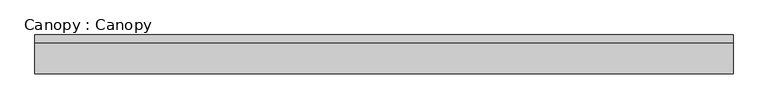
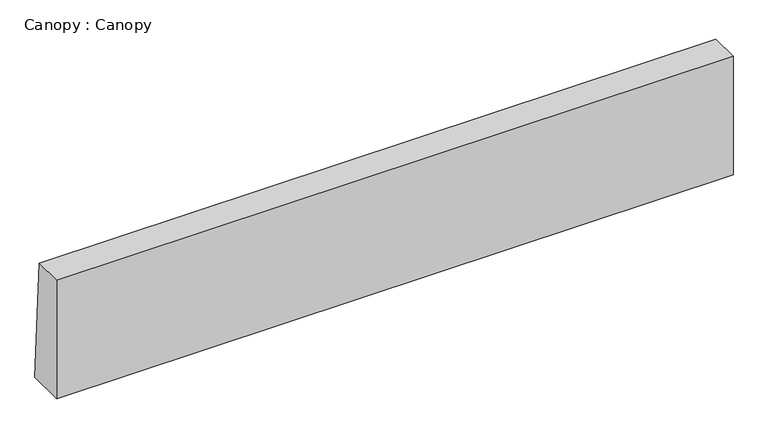
"""IFC4 building model written with IfcOpenShell, lengths in millimetres: proxy geometry, Canopy : Canopy."""

from ifc_helpers import new_model, si_unit, frame, origin, place, context, project, spatial, polyline, outline, extrude, source, transform, mapped, element, save


def canopy_canopy_b27b2f1c(model_context):
    return source(origin(), model_context, "Body", "SweptSolid", [
        extrude(outline(polyline([(150.0, 0.0), (0.0, 0.0), (0.0, 500.0), (120.0, 500.0), (150.0, 0.0)])), frame((-1350.0, 0.0, 0.0), z_axis=(1.0, 0.0, 0.0), x_axis=(0.0, 1.0, 0.0)), (0.0, 0.0, 1.0), 2700.0),
    ])


if __name__ == "__main__":
    model = new_model("IFC4")
    model_context = context("Model", 3, world=origin())
    ifc_project = project(units=[si_unit("LENGTHUNIT", "METRE", prefix="MILLI")], contexts=[model_context])
    site = spatial("IfcSite", under=ifc_project)
    building = spatial("IfcBuilding", under=site)
    placement = place(None, origin())
    canopy_canopy_shape = canopy_canopy_b27b2f1c(model_context)
    element("IfcBuildingElementProxy", 1, Name="Canopy : Canopy", ObjectType="Canopy : Canopy", at=placement, inside=building, context=model_context, shape_type="MappedRepresentation", body=[
        mapped(canopy_canopy_shape, transform((0.0, 0.0, 0.0), x_axis=(1.0, 0.0, 0.0), y_axis=(0.0, 1.0, 0.0), z_axis=(0.0, 0.0, 1.0))),
    ])
    save(model, "model.ifc")

# Revit data of these elements
# Type "Canopy : Canopy"
#   Type Comments = "CV-AG"
#   H_Rebar Ratio = 0.1
#   Canopy Width [instance default] = 1700 mm
#   Canopy Length [instance default] = 1000 mm
#   Canopy L.P = 120 mm
#   Canopy H.P = 150 mm
#   구조재료 = Concrete_f'c=28MPa(Cylender)
#   Default Elevation = 0
# Element 1 (IfcBuildingElementProxy, "Canopy : Canopy")
#   Canopy Width = 2700 mm
#   Canopy Length = 500 mm
#   Materials on its faces: "Concrete_f'c=28MPa(Cylender)"
# Materials
#   "Concrete_f'c=28MPa(Cylender)": class "Concrete", colour RGB 176 176 176, transparency 0, Description = "Reinf. Conc.", Cost = 0, Image = Concrete.Cast-In-Place.Flat.Polished.Grey.jpg
